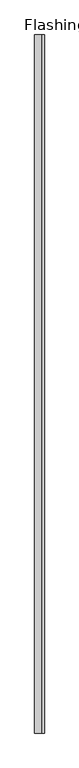
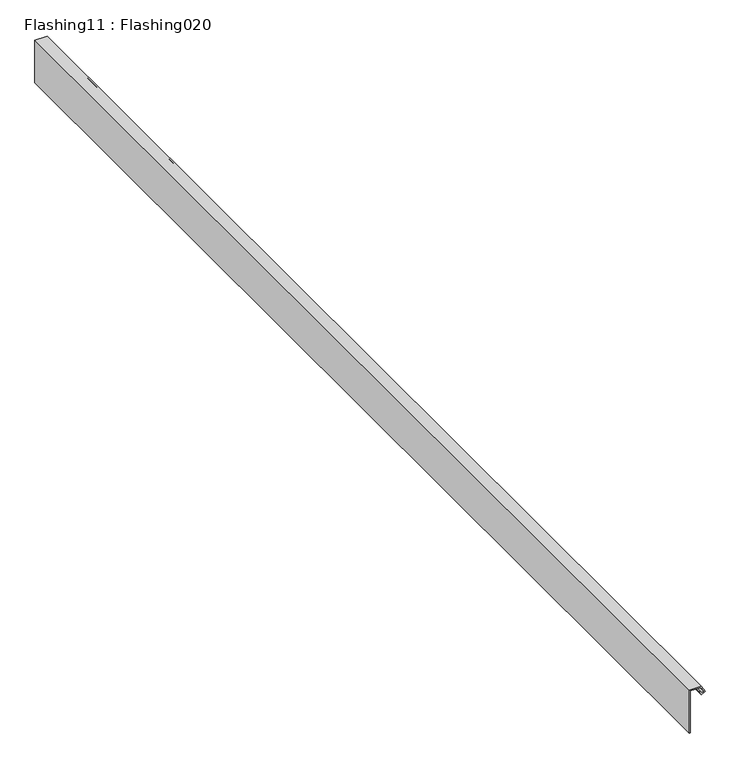
"""IFC4 building model written with IfcOpenShell, lengths in millimetres: proxy geometry, Flashing11 : Flashing020."""

from ifc_helpers import new_model, si_unit, frame, origin, place, context, project, spatial, polyline, outline, extrude, source, transform, mapped, element, save


def flashing11_flashing020_07dce5c2(model_context):
    return source(origin(), model_context, "Body", "SweptSolid", [
        extrude(outline(polyline([(40707.8367188, 16632.328125), (40785.71875, 16632.328125), (40785.71875, 16650.5221509), (40777.2623654, 16655.298745), (40775.2340727, 16652.1607025), (40779.327926, 16649.9538597), (40778.3789063, 16648.1933594), (40772.3789063, 16651.4277344), (40776.6054688, 16657.9667969), (40787.71875, 16651.6894531), (40787.71875, 16630.328125), (40707.8367188, 16630.328125), (40707.8367188, 16632.328125)])), frame((0.0, 7982.1449112, 0.0), z_axis=(0.0, 1.0, 0.0), x_axis=(0.0, 0.0, 1.0)), (0.0, 0.0, 1.0), 2000.0),
    ])


if __name__ == "__main__":
    model = new_model("IFC4")
    model_context = context("Model", 3, world=origin())
    ifc_project = project(units=[si_unit("LENGTHUNIT", "METRE", prefix="MILLI")], contexts=[model_context])
    site = spatial("IfcSite", under=ifc_project)
    building = spatial("IfcBuilding", under=site)
    placement = place(None, origin())
    flashing11_flashing020_shape = flashing11_flashing020_07dce5c2(model_context)
    element("IfcBuildingElementProxy", 1, Name="Flashing11 : Flashing020", ObjectType="Flashing11 : Flashing020", at=placement, inside=building, context=model_context, shape_type="MappedRepresentation", body=[
        mapped(flashing11_flashing020_shape, transform((0.0, 0.0, 0.0), x_axis=(1.0, 0.0, 0.0), y_axis=(0.0, 1.0, 0.0), z_axis=(0.0, 0.0, 1.0))),
    ])
    save(model, "model.ifc")

# Revit data of these elements
# Type "Flashing11 : Flashing020"
#   NameOverride = "Flashing020"
# Element 1 (IfcBuildingElementProxy, "Flashing11 : Flashing020")
#   Materials on its faces: "BRAKE METAL FLASHING TO MATCH STOREFRONT"
# Materials
#   "BRAKE METAL FLASHING TO MATCH STOREFRONT": class "Unassigned", colour RGB 128 128 128, transparency 0, Cost = 0
